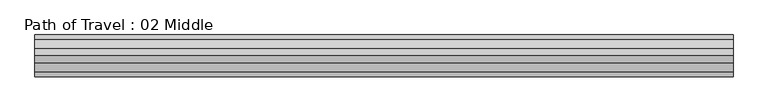
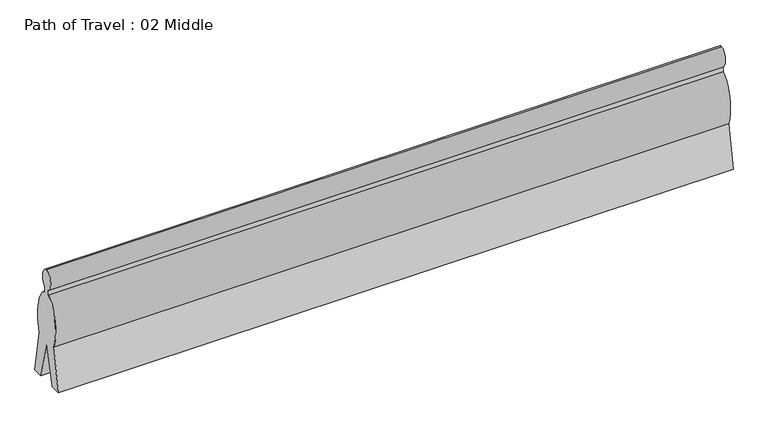
"""IFC4 building model written with IfcOpenShell, lengths in millimetres: proxy geometry, Path of Travel : 02 Middle."""

from ifc_helpers import new_model, si_unit, point, frame, origin, place, context, project, spatial, ellipse_curve, trimmed, source, transform, mapped, element, save
from ifc_brep_helpers import plane_surface, extruded_surface, advanced_brep


def path_of_travel_02_middle_85298eeb(model_context):
    return source(origin(), model_context, "Body", "AdvancedBrep", [
        advanced_brep(
        [(227.5554837, 0.0, 1727.2), (227.5554837, 42.9018657, 1436.6534209), (227.5554837, 42.9018657, 1363.4763406), (227.5554837, 184.1186263, 643.4144547), (227.5554837, 297.5699544, 0.0), (227.5554837, 145.6574193, 0.0), (227.5554837, 0.0, 584.2), (227.5554837, -145.6574193, 0.0), (227.5554837, -297.5699544, 0.0), (227.5554837, -184.1186263, 643.4144547), (227.5554837, -42.9018657, 1363.4763406), (227.5554837, -42.9018657, 1436.6534209), (10133.5554837, 0.0, 1727.2), (10133.5554837, -42.9018657, 1436.6534209), (10133.5554837, -42.9018657, 1363.4763406), (10133.5554837, -184.1186263, 643.4144547), (10133.5554837, -297.5699544, 0.0), (10133.5554837, -145.6574193, 0.0), (10133.5554837, 0.0, 584.2), (10133.5554837, 145.6574193, 0.0), (10133.5554837, 297.5699544, 0.0), (10133.5554837, 184.1186263, 643.4144547), (10133.5554837, 42.9018657, 1363.4763406), (10133.5554837, 42.9018657, 1436.6534209)],
        [
            (0, 1, ellipse_curve(frame((227.5554837, 0.0, 1574.8), z_axis=(-1.0, 0.0, 0.0), x_axis=(0.0, 0.0, 1.0)), 152.4, 101.6)),
            (1, 2),
            (2, 3, ellipse_curve(frame((227.5554837, 0.0, 914.4), z_axis=(-1.0, 0.0, 0.0), x_axis=(0.0, 0.0, -1.0)), 457.2, 228.6)),
            (3, 4),
            (4, 5),
            (5, 6),
            (6, 7),
            (7, 8),
            (8, 9),
            (9, 10, ellipse_curve(frame((227.5554837, 0.0, 914.4), z_axis=(-1.0, 0.0, 0.0), x_axis=(0.0, 0.0, -1.0)), 457.2, 228.6)),
            (10, 11),
            (11, 0, ellipse_curve(frame((227.5554837, 0.0, 1574.8), z_axis=(-1.0, 0.0, 0.0), x_axis=(0.0, 0.0, 1.0)), 152.4, 101.6)),
            (12, 13, ellipse_curve(frame((10133.5554837, 0.0, 1574.8), z_axis=(1.0, 0.0, 0.0), x_axis=(0.0, 0.0, 1.0)), 152.4, 101.6)),
            (13, 14),
            (14, 15, ellipse_curve(frame((10133.5554837, 0.0, 914.4), z_axis=(1.0, 0.0, 0.0), x_axis=(0.0, 0.0, -1.0)), 457.2, 228.6)),
            (15, 16),
            (16, 17),
            (17, 18),
            (18, 19),
            (19, 20),
            (20, 21),
            (21, 22, ellipse_curve(frame((10133.5554837, 0.0, 914.4), z_axis=(1.0, 0.0, 0.0), x_axis=(0.0, 0.0, -1.0)), 457.2, 228.6)),
            (22, 23),
            (23, 12, ellipse_curve(frame((10133.5554837, 0.0, 1574.8), z_axis=(1.0, 0.0, 0.0), x_axis=(0.0, 0.0, 1.0)), 152.4, 101.6)),
            (0, 12),
            (23, 1),
            (22, 2),
            (21, 3),
            (20, 4),
            (19, 5),
            (18, 6),
            (17, 7),
            (16, 8),
            (15, 9),
            (14, 10),
            (13, 11),
        ],
        [
            plane_surface(frame((227.5554837, 0.0, 0.0), z_axis=(-1.0, 0.0, 0.0), x_axis=(0.0, 0.0, 1.0))),
            plane_surface(frame((10133.5554837, 0.0, 0.0), z_axis=(1.0, 0.0, 0.0), x_axis=(0.0, 0.0, 1.0))),
            extruded_surface(trimmed(ellipse_curve(frame((10133.5554837, 0.0, 1574.8), z_axis=(-1.0, 0.0, 0.0), x_axis=(0.0, 0.0, 1.0)), 152.4, 101.6), [point((10133.5554837, 0.0, 1727.2))], [point((10133.5554837, 42.9018657, 1436.6534209))], True, "CARTESIAN"), (-9906.0, 0.0, 0.0), 9906.0),
            plane_surface(frame((227.5554837, 42.9018657, 1436.6534209), z_axis=(0.0, 1.0, 0.0), x_axis=(1.0, 0.0, 0.0))),
            extruded_surface(trimmed(ellipse_curve(frame((10133.5554837, 0.0, 914.4), z_axis=(-1.0, 0.0, 0.0), x_axis=(0.0, 0.0, -1.0)), 457.2, 228.6), [point((10133.5554837, 42.9018657, 1363.4763406))], [point((10133.5554837, 184.1186263, 643.4144547))], True, "CARTESIAN"), (-9906.0, 0.0, 0.0), 9906.0),
            plane_surface(frame((227.5554837, 184.1186263, 643.4144547), z_axis=(0.0, 0.9848077530122078, 0.17364817766693205), x_axis=(1.0, 0.0, 0.0))),
            plane_surface(frame((227.5554837, 297.5699544, 0.0), z_axis=(0.0, 0.0, -1.0), x_axis=(1.0, 0.0, 0.0))),
            plane_surface(frame((227.5554837, 145.6574193, 0.0), z_axis=(0.0, -0.9702957262760199, -0.2419218955995739), x_axis=(1.0, 0.0, 0.0))),
            plane_surface(frame((227.5554837, 0.0, 584.2), z_axis=(0.0, 0.9702957262759961, -0.24192189559966923), x_axis=(1.0, 0.0, 0.0))),
            plane_surface(frame((227.5554837, -145.6574193, 0.0), z_axis=(0.0, 0.0, -1.0), x_axis=(1.0, 0.0, 0.0))),
            plane_surface(frame((227.5554837, -297.5699544, 0.0), z_axis=(0.0, -0.984807753012208, 0.17364817766693066), x_axis=(1.0, 0.0, 0.0))),
            extruded_surface(trimmed(ellipse_curve(frame((10133.5554837, 0.0, 914.4), z_axis=(-1.0, 0.0, 0.0), x_axis=(0.0, 0.0, -1.0)), 457.2, 228.6), [point((10133.5554837, -184.1186263, 643.4144547))], [point((10133.5554837, -42.9018657, 1363.4763406))], True, "CARTESIAN"), (-9906.0, 0.0, 0.0), 9906.0),
            plane_surface(frame((227.5554837, -42.9018657, 1363.4763406), z_axis=(0.0, -1.0, 0.0), x_axis=(1.0, 0.0, 0.0))),
            extruded_surface(trimmed(ellipse_curve(frame((10133.5554837, 0.0, 1574.8), z_axis=(-1.0, 0.0, 0.0), x_axis=(0.0, 0.0, 1.0)), 152.4, 101.6), [point((10133.5554837, -42.9018657, 1436.6534209))], [point((10133.5554837, 0.0, 1727.2))], True, "CARTESIAN"), (-9906.0, 0.0, 0.0), 9906.0),
        ],
        [
            (0, [[1, 2, 3, 4, 5, 6, 7, 8, 9, 10, 11, 12]]),
            (1, [[13, 14, 15, 16, 17, 18, 19, 20, 21, 22, 23, 24]]),
            (2, [[-1, 25, -24, 26]]),
            (3, [[-2, -26, -23, 27]]),
            (4, [[-3, -27, -22, 28]]),
            (5, [[-4, -28, -21, 29]]),
            (6, [[-5, -29, -20, 30]]),
            (7, [[-6, -30, -19, 31]]),
            (8, [[-7, -31, -18, 32]]),
            (9, [[-8, -32, -17, 33]]),
            (10, [[-9, -33, -16, 34]]),
            (11, [[-10, -34, -15, 35]]),
            (12, [[-11, -35, -14, 36]]),
            (13, [[-12, -36, -13, -25]]),
        ],
    ),
    ])


if __name__ == "__main__":
    model = new_model("IFC4")
    model_context = context("Model", 3, world=origin())
    ifc_project = project(units=[si_unit("LENGTHUNIT", "METRE", prefix="MILLI")], contexts=[model_context])
    site = spatial("IfcSite", under=ifc_project)
    building = spatial("IfcBuilding", under=site)
    placement = place(None, origin())
    path_of_travel_02_middle_shape = path_of_travel_02_middle_85298eeb(model_context)
    element("IfcBuildingElementProxy", 1, Name="Path of Travel : 02 Middle", ObjectType="Path of Travel : 02 Middle", at=placement, inside=building, context=model_context, shape_type="MappedRepresentation", body=[
        mapped(path_of_travel_02_middle_shape, transform((0.0, 0.0, 0.0), x_axis=(1.0, 0.0, 0.0), y_axis=(0.0, 1.0, 0.0), z_axis=(0.0, 0.0, 1.0))),
    ])
    save(model, "model.ifc")

# Revit data of these elements
# Type "Path of Travel : 02 Middle"
#   Path of Egress [instance default] = 4' - 0"
#   built-in parameter 1001306 [instance default] = 4 (stored number, unit not read)
#   Dot at Start = no
#   Arrow in Middle = yes
#   Arrow at End = no
#   Egress Path = none
# Element 1 (IfcBuildingElementProxy, "Path of Travel : 02 Middle")
#   Path of Egress = 32' - 6"
#   built-in parameter 1001306 = 32.5 (stored number, unit not read)
#   Materials on its faces: "Egress Path Solid"
# Materials
#   "Egress Path Solid": class "Unassigned", colour RGB 255 128 64, transparency 0.75, Comments = "Rendering appearance not upgraded "
